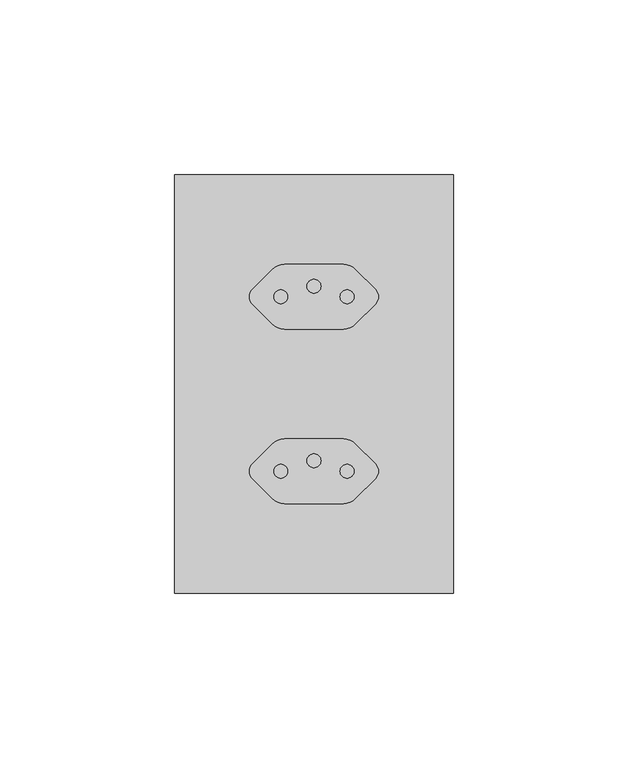
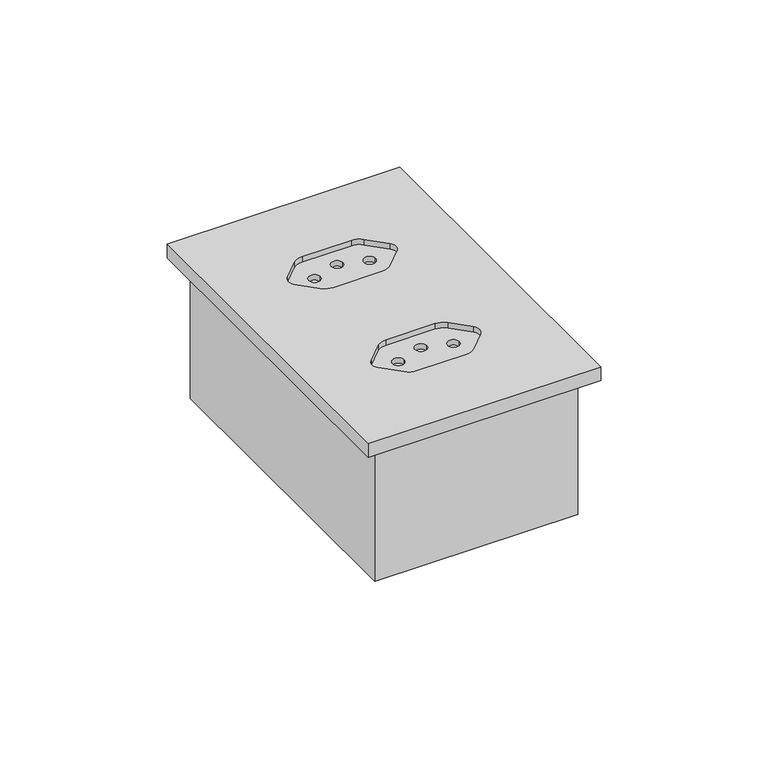
"""IFC4 building model written with IfcOpenShell, lengths in millimetres: proxy geometry, CAIXA VERTICE V7 : Tomada 10A 2s."""

from ifc_helpers import new_model, si_unit, frame, origin, place, context, project, spatial, polyline, circle_curve, faceted_brep, source, transform, mapped, element, save
from ifc_brep_helpers import plane_surface, revolved_surface, advanced_brep


def electrical_fixtures_a300802b(model_context):
    return source(origin(), model_context, "Body", "SolidModel", [
        faceted_brep([(33.0, 247.0, -48.0), (33.0, 353.0, -48.0), (-33.0, 353.0, -48.0), (-33.0, 247.0, -48.0), (35.0, 355.0, -50.0), (35.0, 245.0, -50.0), (-35.0, 245.0, -50.0), (-35.0, 355.0, -50.0), (-35.0, 355.0, 0.0), (35.0, 355.0, 0.0), (-35.0, 245.0, 0.0), (35.0, 245.0, 0.0), (33.0, 353.0, 0.0), (33.0, 247.0, 0.0), (-33.0, 247.0, 0.0), (-33.0, 353.0, 0.0)], [[[0, 1, 2, 3]], [[4, 5, 6, 7]], [[4, 7, 8, 9]], [[8, 7, 6, 10]], [[10, 6, 5, 11]], [[11, 5, 4, 9]], [[9, 8, 10, 11], [12, 13, 14, 15]], [[13, 12, 1, 0]], [[14, 13, 0, 3]], [[15, 14, 3, 2]], [[12, 15, 2, 1]]]),
        advanced_brep(
        [(40.0, 360.0, 5.0), (-40.0, 360.0, 5.0), (-40.0, 240.0, 5.0), (40.0, 240.0, 5.0), (8.4215729, 315.75, 5.0), (-8.4215729, 315.75, 5.0), (-11.9571068, 317.2144661, 5.0), (-17.6213203, 322.8786797, 5.0), (-17.6213203, 327.1213203, 5.0), (-11.9571068, 332.7855339, 5.0), (-8.4215729, 334.25, 5.0), (8.4215729, 334.25, 5.0), (11.9571068, 332.7855339, 5.0), (17.6213203, 327.1213203, 5.0), (17.6213203, 322.8786797, 5.0), (11.9571068, 317.2144661, 5.0), (8.4215729, 265.75, 5.0), (-8.4215729, 265.75, 5.0), (-11.9571068, 267.2144661, 5.0), (-17.6213203, 272.8786797, 5.0), (-17.6213203, 277.1213203, 5.0), (-11.9571068, 282.7855339, 5.0), (-8.4215729, 284.25, 5.0), (8.4215729, 284.25, 5.0), (11.9571068, 282.7855339, 5.0), (17.6213203, 277.1213203, 5.0), (17.6213203, 272.8786797, 5.0), (11.9571068, 267.2144661, 5.0), (-40.0, 360.0, 0.0), (40.0, 360.0, 0.0), (40.0, 240.0, 0.0), (-40.0, 240.0, 0.0), (8.4215729, 315.75, 3.0), (11.9571068, 317.2144661, 3.0), (17.6213203, 322.8786797, 3.0), (17.6213203, 327.1213203, 3.0), (11.9571068, 332.7855339, 3.0), (8.4215729, 334.25, 3.0), (-8.4215729, 334.25, 3.0), (-11.9571068, 332.7855339, 3.0), (-17.6213203, 327.1213203, 3.0), (-17.6213203, 322.8786797, 3.0), (-11.9571068, 317.2144661, 3.0), (-8.4215729, 315.75, 3.0), (-7.5, 325.0, 3.0), (-11.5, 325.0, 3.0), (11.5, 325.0, 3.0), (7.5, 325.0, 3.0), (2.0, 328.0, 3.0), (-2.0, 328.0, 3.0), (-11.5, 325.0, 1.0), (-7.5, 325.0, 1.0), (7.5, 325.0, 1.0), (11.5, 325.0, 1.0), (-2.0, 328.0, 1.0), (2.0, 328.0, 1.0), (8.4215729, 265.75, 3.0), (11.9571068, 267.2144661, 3.0), (17.6213203, 272.8786797, 3.0), (17.6213203, 277.1213203, 3.0), (11.9571068, 282.7855339, 3.0), (8.4215729, 284.25, 3.0), (-8.4215729, 284.25, 3.0), (-11.9571068, 282.7855339, 3.0), (-17.6213203, 277.1213203, 3.0), (-17.6213203, 272.8786797, 3.0), (-11.9571068, 267.2144661, 3.0), (-8.4215729, 265.75, 3.0), (-7.5, 275.0, 3.0), (-11.5, 275.0, 3.0), (11.5, 275.0, 3.0), (7.5, 275.0, 3.0), (2.0, 278.0, 3.0), (-2.0, 278.0, 3.0), (-11.5, 275.0, 1.0), (-7.5, 275.0, 1.0), (7.5, 275.0, 1.0), (11.5, 275.0, 1.0), (-2.0, 278.0, 1.0), (2.0, 278.0, 1.0)],
        [
            (0, 1),
            (1, 2),
            (2, 3),
            (3, 0),
            (4, 5),
            (5, 6, circle_curve(frame((-8.4215729, 320.75, 5.0), z_axis=(0.0, 0.0, -1.0), x_axis=(-1.0, 0.0, 0.0)), 5.0)),
            (6, 7),
            (7, 8, circle_curve(frame((-15.5, 325.0, 5.0), z_axis=(0.0, 0.0, -1.0), x_axis=(-1.0, 0.0, 0.0)), 3.0)),
            (8, 9),
            (9, 10, circle_curve(frame((-8.4215729, 329.25, 5.0), z_axis=(0.0, 0.0, -1.0), x_axis=(-1.0, 0.0, 0.0)), 5.0)),
            (10, 11),
            (11, 12, circle_curve(frame((8.4215729, 329.25, 5.0), z_axis=(0.0, 0.0, -1.0), x_axis=(-1.0, 0.0, 0.0)), 5.0)),
            (12, 13),
            (13, 14, circle_curve(frame((15.5, 325.0, 5.0), z_axis=(0.0, 0.0, -1.0), x_axis=(-1.0, 0.0, 0.0)), 3.0)),
            (14, 15),
            (15, 4, circle_curve(frame((8.4215729, 320.75, 5.0), z_axis=(0.0, 0.0, -1.0), x_axis=(-1.0, 0.0, 0.0)), 5.0)),
            (16, 17),
            (17, 18, circle_curve(frame((-8.4215729, 270.75, 5.0), z_axis=(0.0, 0.0, -1.0), x_axis=(-1.0, 0.0, 0.0)), 5.0)),
            (18, 19),
            (19, 20, circle_curve(frame((-15.5, 275.0, 5.0), z_axis=(0.0, 0.0, -1.0), x_axis=(-1.0, 0.0, 0.0)), 3.0)),
            (20, 21),
            (21, 22, circle_curve(frame((-8.4215729, 279.25, 5.0), z_axis=(0.0, 0.0, -1.0), x_axis=(-1.0, 0.0, 0.0)), 5.0)),
            (22, 23),
            (23, 24, circle_curve(frame((8.4215729, 279.25, 5.0), z_axis=(0.0, 0.0, -1.0), x_axis=(-1.0, 0.0, 0.0)), 5.0)),
            (24, 25),
            (25, 26, circle_curve(frame((15.5, 275.0, 5.0), z_axis=(0.0, 0.0, -1.0), x_axis=(-1.0, 0.0, 0.0)), 3.0)),
            (26, 27),
            (27, 16, circle_curve(frame((8.4215729, 270.75, 5.0), z_axis=(0.0, 0.0, -1.0), x_axis=(-1.0, 0.0, 0.0)), 5.0)),
            (28, 29),
            (29, 30),
            (30, 31),
            (31, 28),
            (0, 29),
            (28, 1),
            (31, 2),
            (30, 3),
            (32, 33, circle_curve(frame((8.4215729, 320.75, 3.0), z_axis=(0.0, 0.0, 1.0), x_axis=(-1.0, 0.0, 0.0)), 5.0)),
            (33, 34),
            (34, 35, circle_curve(frame((15.5, 325.0, 3.0), z_axis=(0.0, 0.0, 1.0), x_axis=(-1.0, 0.0, 0.0)), 3.0)),
            (35, 36),
            (36, 37, circle_curve(frame((8.4215729, 329.25, 3.0), z_axis=(0.0, 0.0, 1.0), x_axis=(-1.0, 0.0, 0.0)), 5.0)),
            (37, 38),
            (38, 39, circle_curve(frame((-8.4215729, 329.25, 3.0), z_axis=(0.0, 0.0, 1.0), x_axis=(-1.0, 0.0, 0.0)), 5.0)),
            (39, 40),
            (40, 41, circle_curve(frame((-15.5, 325.0, 3.0), z_axis=(0.0, 0.0, 1.0), x_axis=(-1.0, 0.0, 0.0)), 3.0)),
            (41, 42),
            (42, 43, circle_curve(frame((-8.4215729, 320.75, 3.0), z_axis=(0.0, 0.0, 1.0), x_axis=(-1.0, 0.0, 0.0)), 5.0)),
            (43, 32),
            (44, 45, circle_curve(frame((-9.5, 325.0, 3.0), z_axis=(0.0, 0.0, -1.0), x_axis=(1.0, 2.301812013077709e-12, 0.0)), 2.0)),
            (45, 44, circle_curve(frame((-9.5, 325.0, 3.0), z_axis=(0.0, 0.0, -1.0), x_axis=(1.0, 2.301812013077709e-12, 0.0)), 2.0)),
            (46, 47, circle_curve(frame((9.5, 325.0, 3.0), z_axis=(0.0, 0.0, -1.0), x_axis=(1.0, 2.301812013077709e-12, 0.0)), 2.0)),
            (47, 46, circle_curve(frame((9.5, 325.0, 3.0), z_axis=(0.0, 0.0, -1.0), x_axis=(1.0, 2.301812013077709e-12, 0.0)), 2.0)),
            (48, 49, circle_curve(frame((0.0, 328.0, 3.0), z_axis=(0.0, 0.0, -1.0), x_axis=(1.0, 2.301812013077709e-12, 0.0)), 2.0)),
            (49, 48, circle_curve(frame((0.0, 328.0, 3.0), z_axis=(0.0, 0.0, -1.0), x_axis=(1.0, 2.301812013077709e-12, 0.0)), 2.0)),
            (43, 5),
            (4, 32),
            (42, 6),
            (41, 7),
            (40, 8),
            (39, 9),
            (38, 10),
            (37, 11),
            (36, 12),
            (35, 13),
            (34, 14),
            (33, 15),
            (50, 51, circle_curve(frame((-9.5, 325.0, 1.0), z_axis=(0.0, 0.0, 1.0), x_axis=(1.0, 2.301812013077709e-12, 0.0)), 2.0)),
            (51, 50, circle_curve(frame((-9.5, 325.0, 1.0), z_axis=(0.0, 0.0, 1.0), x_axis=(1.0, 2.301812013077709e-12, 0.0)), 2.0)),
            (52, 53, circle_curve(frame((9.5, 325.0, 1.0), z_axis=(0.0, 0.0, 1.0), x_axis=(1.0, 2.301812013077709e-12, 0.0)), 2.0)),
            (53, 52, circle_curve(frame((9.5, 325.0, 1.0), z_axis=(0.0, 0.0, 1.0), x_axis=(1.0, 2.301812013077709e-12, 0.0)), 2.0)),
            (54, 55, circle_curve(frame((0.0, 328.0, 1.0), z_axis=(0.0, 0.0, 1.0), x_axis=(1.0, 2.301812013077709e-12, 0.0)), 2.0)),
            (55, 54, circle_curve(frame((0.0, 328.0, 1.0), z_axis=(0.0, 0.0, 1.0), x_axis=(1.0, 2.301812013077709e-12, 0.0)), 2.0)),
            (44, 51),
            (50, 45),
            (46, 53),
            (52, 47),
            (48, 55),
            (54, 49),
            (56, 57, circle_curve(frame((8.4215729, 270.75, 3.0), z_axis=(0.0, 0.0, 1.0), x_axis=(-1.0, 0.0, 0.0)), 5.0)),
            (57, 58),
            (58, 59, circle_curve(frame((15.5, 275.0, 3.0), z_axis=(0.0, 0.0, 1.0), x_axis=(-1.0, 0.0, 0.0)), 3.0)),
            (59, 60),
            (60, 61, circle_curve(frame((8.4215729, 279.25, 3.0), z_axis=(0.0, 0.0, 1.0), x_axis=(-1.0, 0.0, 0.0)), 5.0)),
            (61, 62),
            (62, 63, circle_curve(frame((-8.4215729, 279.25, 3.0), z_axis=(0.0, 0.0, 1.0), x_axis=(-1.0, 0.0, 0.0)), 5.0)),
            (63, 64),
            (64, 65, circle_curve(frame((-15.5, 275.0, 3.0), z_axis=(0.0, 0.0, 1.0), x_axis=(-1.0, 0.0, 0.0)), 3.0)),
            (65, 66),
            (66, 67, circle_curve(frame((-8.4215729, 270.75, 3.0), z_axis=(0.0, 0.0, 1.0), x_axis=(-1.0, 0.0, 0.0)), 5.0)),
            (67, 56),
            (68, 69, circle_curve(frame((-9.5, 275.0, 3.0), z_axis=(0.0, 0.0, -1.0), x_axis=(1.0, 2.301812013077709e-12, 0.0)), 2.0)),
            (69, 68, circle_curve(frame((-9.5, 275.0, 3.0), z_axis=(0.0, 0.0, -1.0), x_axis=(1.0, 2.301812013077709e-12, 0.0)), 2.0)),
            (70, 71, circle_curve(frame((9.5, 275.0, 3.0), z_axis=(0.0, 0.0, -1.0), x_axis=(1.0, 2.301812013077709e-12, 0.0)), 2.0)),
            (71, 70, circle_curve(frame((9.5, 275.0, 3.0), z_axis=(0.0, 0.0, -1.0), x_axis=(1.0, 2.301812013077709e-12, 0.0)), 2.0)),
            (72, 73, circle_curve(frame((0.0, 278.0, 3.0), z_axis=(0.0, 0.0, -1.0), x_axis=(1.0, 2.301812013077709e-12, 0.0)), 2.0)),
            (73, 72, circle_curve(frame((0.0, 278.0, 3.0), z_axis=(0.0, 0.0, -1.0), x_axis=(1.0, 2.301812013077709e-12, 0.0)), 2.0)),
            (67, 17),
            (16, 56),
            (66, 18),
            (65, 19),
            (64, 20),
            (63, 21),
            (62, 22),
            (61, 23),
            (60, 24),
            (59, 25),
            (58, 26),
            (57, 27),
            (74, 75, circle_curve(frame((-9.5, 275.0, 1.0), z_axis=(0.0, 0.0, 1.0), x_axis=(1.0, 2.301812013077709e-12, 0.0)), 2.0)),
            (75, 74, circle_curve(frame((-9.5, 275.0, 1.0), z_axis=(0.0, 0.0, 1.0), x_axis=(1.0, 2.301812013077709e-12, 0.0)), 2.0)),
            (76, 77, circle_curve(frame((9.5, 275.0, 1.0), z_axis=(0.0, 0.0, 1.0), x_axis=(1.0, 2.301812013077709e-12, 0.0)), 2.0)),
            (77, 76, circle_curve(frame((9.5, 275.0, 1.0), z_axis=(0.0, 0.0, 1.0), x_axis=(1.0, 2.301812013077709e-12, 0.0)), 2.0)),
            (78, 79, circle_curve(frame((0.0, 278.0, 1.0), z_axis=(0.0, 0.0, 1.0), x_axis=(1.0, 2.301812013077709e-12, 0.0)), 2.0)),
            (79, 78, circle_curve(frame((0.0, 278.0, 1.0), z_axis=(0.0, 0.0, 1.0), x_axis=(1.0, 2.301812013077709e-12, 0.0)), 2.0)),
            (68, 75),
            (74, 69),
            (70, 77),
            (76, 71),
            (72, 79),
            (78, 73),
        ],
        [
            plane_surface(frame((-60.0, 360.0, 5.0), z_axis=(0.0, 0.0, 1.0), x_axis=(-1.0, 0.0, 0.0))),
            plane_surface(frame((-60.0, 360.0, 0.0), z_axis=(0.0, 0.0, -1.0), x_axis=(1.0, 0.0, 0.0))),
            plane_surface(frame((40.0, 360.0, 5.0), z_axis=(0.0, 1.0, 0.0), x_axis=(0.0, 0.0, -1.0))),
            plane_surface(frame((-40.0, 360.0, 5.0), z_axis=(-1.0, 0.0, 0.0), x_axis=(0.0, 0.0, -1.0))),
            plane_surface(frame((-40.0, 240.0, 5.0), z_axis=(0.0, -1.0, 0.0), x_axis=(0.0, 0.0, -1.0))),
            plane_surface(frame((40.0, 240.0, 5.0), z_axis=(1.0, 0.0, 0.0), x_axis=(0.0, 0.0, -1.0))),
            plane_surface(frame((3.4215729, 320.75, 3.0), z_axis=(0.0, 0.0, 1.0), x_axis=(0.0, 1.0, 0.0))),
            plane_surface(frame((-8.4215729, 315.75, 5.0), z_axis=(0.0, 1.0, 0.0), x_axis=(0.0, 0.0, -1.0))),
            revolved_surface(polyline([(-13.4215729, 320.75, 5.0), (-13.4215729, 320.75, 3.0)]), (-8.4215729, 320.75, 3.0), (0.0, 0.0, 1.0)),
            plane_surface(frame((-17.6213203, 322.8786797, 5.0), z_axis=(0.7071067811865045, 0.7071067811865905, 0.0), x_axis=(0.0, 0.0, -1.0))),
            revolved_surface(polyline([(-18.5, 325.0, 5.0), (-18.5, 325.0, 3.0)]), (-15.5, 325.0, 3.0), (0.0, 0.0, 1.0)),
            plane_surface(frame((-11.9571068, 332.7855339, 5.0), z_axis=(0.7071067811865515, -0.7071067811865437, 0.0), x_axis=(0.0, 0.0, -1.0))),
            revolved_surface(polyline([(-13.4215729, 329.25, 5.0), (-13.4215729, 329.25, 3.0)]), (-8.4215729, 329.25, 3.0), (0.0, 0.0, 1.0)),
            plane_surface(frame((8.4215729, 334.25, 5.0), z_axis=(0.0, -1.0, 0.0), x_axis=(0.0, 0.0, -1.0))),
            revolved_surface(polyline([(3.4215728999999993, 329.25, 5.0), (3.4215728999999993, 329.25, 3.0)]), (8.4215729, 329.25, 3.0), (0.0, 0.0, 1.0)),
            plane_surface(frame((17.6213203, 327.1213203, 5.0), z_axis=(-0.7071067811865307, -0.7071067811865643, 0.0), x_axis=(0.0, 0.0, -1.0))),
            revolved_surface(polyline([(12.5, 325.0, 5.0), (12.5, 325.0, 3.0)]), (15.5, 325.0, 3.0), (0.0, 0.0, 1.0)),
            plane_surface(frame((11.9571068, 317.2144661, 5.0), z_axis=(-0.7071067811865893, 0.7071067811865058, 0.0), x_axis=(0.0, 0.0, -1.0))),
            revolved_surface(polyline([(3.4215728999999993, 320.75, 5.0), (3.4215728999999993, 320.75, 3.0)]), (8.4215729, 320.75, 3.0), (0.0, 0.0, 1.0)),
            plane_surface(frame((-7.5, 325.0, 1.0), z_axis=(0.0, 0.0, 1.0), x_axis=(2.301812013077709e-12, -1.0, 0.0))),
            revolved_surface(polyline([(-7.5, 325.0000000000046, 3.0), (-7.5, 325.0000000000046, 1.0)]), (-9.5, 325.0, 1.0), (0.0, 0.0, 1.0)),
            revolved_surface(polyline([(11.5, 325.0000000000046, 3.0), (11.5, 325.0000000000046, 1.0)]), (9.5, 325.0, 5.0), (0.0, 0.0, 1.0)),
            revolved_surface(polyline([(2.0, 328.0000000000046, 3.0), (2.0, 328.0000000000046, 1.0)]), (0.0, 328.0, 5.0), (0.0, 0.0, 1.0)),
            plane_surface(frame((3.4215729, 270.75, 3.0), z_axis=(0.0, 0.0, 1.0), x_axis=(0.0, 1.0, 0.0))),
            plane_surface(frame((-8.4215729, 265.75, 5.0), z_axis=(0.0, 1.0, 0.0), x_axis=(0.0, 0.0, -1.0))),
            revolved_surface(polyline([(-13.4215729, 270.75, 5.0), (-13.4215729, 270.75, 3.0)]), (-8.4215729, 270.75, 3.0), (0.0, 0.0, 1.0)),
            plane_surface(frame((-17.6213203, 272.8786797, 5.0), z_axis=(0.7071067811865045, 0.7071067811865905, 0.0), x_axis=(0.0, 0.0, -1.0))),
            revolved_surface(polyline([(-18.5, 275.0, 5.0), (-18.5, 275.0, 3.0)]), (-15.5, 275.0, 3.0), (0.0, 0.0, 1.0)),
            plane_surface(frame((-11.9571068, 282.7855339, 5.0), z_axis=(0.7071067811865515, -0.7071067811865437, 0.0), x_axis=(0.0, 0.0, -1.0))),
            revolved_surface(polyline([(-13.4215729, 279.25, 5.0), (-13.4215729, 279.25, 3.0)]), (-8.4215729, 279.25, 3.0), (0.0, 0.0, 1.0)),
            plane_surface(frame((8.4215729, 284.25, 5.0), z_axis=(0.0, -1.0, 0.0), x_axis=(0.0, 0.0, -1.0))),
            revolved_surface(polyline([(3.4215728999999993, 279.25, 5.0), (3.4215728999999993, 279.25, 3.0)]), (8.4215729, 279.25, 3.0), (0.0, 0.0, 1.0)),
            plane_surface(frame((17.6213203, 277.1213203, 5.0), z_axis=(-0.7071067811865307, -0.7071067811865643, 0.0), x_axis=(0.0, 0.0, -1.0))),
            revolved_surface(polyline([(12.5, 275.0, 5.0), (12.5, 275.0, 3.0)]), (15.5, 275.0, 3.0), (0.0, 0.0, 1.0)),
            plane_surface(frame((11.9571068, 267.2144661, 5.0), z_axis=(-0.7071067811865893, 0.7071067811865058, 0.0), x_axis=(0.0, 0.0, -1.0))),
            revolved_surface(polyline([(3.4215728999999993, 270.75, 5.0), (3.4215728999999993, 270.75, 3.0)]), (8.4215729, 270.75, 3.0), (0.0, 0.0, 1.0)),
            plane_surface(frame((-7.5, 275.0, 1.0), z_axis=(0.0, 0.0, 1.0), x_axis=(2.301812013077709e-12, -1.0, 0.0))),
            revolved_surface(polyline([(-7.5, 275.0000000000046, 3.0), (-7.5, 275.0000000000046, 1.0)]), (-9.5, 275.0, 1.0), (0.0, 0.0, 1.0)),
            revolved_surface(polyline([(11.5, 275.0000000000046, 3.0), (11.5, 275.0000000000046, 1.0)]), (9.5, 275.0, 5.0), (0.0, 0.0, 1.0)),
            revolved_surface(polyline([(2.0, 278.0000000000046, 3.0), (2.0, 278.0000000000046, 1.0)]), (0.0, 278.0, 5.0), (0.0, 0.0, 1.0)),
        ],
        [
            (0, [[1, 2, 3, 4], [5, 6, 7, 8, 9, 10, 11, 12, 13, 14, 15, 16], [17, 18, 19, 20, 21, 22, 23, 24, 25, 26, 27, 28]]),
            (1, [[29, 30, 31, 32]]),
            (2, [[-1, 33, -29, 34]]),
            (3, [[-2, -34, -32, 35]]),
            (4, [[-3, -35, -31, 36]]),
            (5, [[-4, -36, -30, -33]]),
            (6, [[37, 38, 39, 40, 41, 42, 43, 44, 45, 46, 47, 48], [49, 50], [51, 52], [53, 54]]),
            (7, [[-48, 55, -5, 56]]),
            (8, [[-47, 57, -6, -55]]),
            (9, [[-46, 58, -7, -57]]),
            (10, [[-45, 59, -8, -58]]),
            (11, [[-44, 60, -9, -59]]),
            (12, [[-43, 61, -10, -60]]),
            (13, [[-42, 62, -11, -61]]),
            (14, [[-41, 63, -12, -62]]),
            (15, [[-40, 64, -13, -63]]),
            (16, [[-39, 65, -14, -64]]),
            (17, [[-38, 66, -15, -65]]),
            (18, [[-37, -56, -16, -66]]),
            (19, [[67, 68]]),
            (19, [[69, 70]]),
            (19, [[71, 72]]),
            (20, [[-49, 73, -67, 74]]),
            (20, [[-50, -74, -68, -73]]),
            (21, [[-51, 75, -69, 76]]),
            (21, [[-52, -76, -70, -75]]),
            (22, [[-53, 77, -71, 78]]),
            (22, [[-54, -78, -72, -77]]),
            (23, [[79, 80, 81, 82, 83, 84, 85, 86, 87, 88, 89, 90], [91, 92], [93, 94], [95, 96]]),
            (24, [[-90, 97, -17, 98]]),
            (25, [[-89, 99, -18, -97]]),
            (26, [[-88, 100, -19, -99]]),
            (27, [[-87, 101, -20, -100]]),
            (28, [[-86, 102, -21, -101]]),
            (29, [[-85, 103, -22, -102]]),
            (30, [[-84, 104, -23, -103]]),
            (31, [[-83, 105, -24, -104]]),
            (32, [[-82, 106, -25, -105]]),
            (33, [[-81, 107, -26, -106]]),
            (34, [[-80, 108, -27, -107]]),
            (35, [[-79, -98, -28, -108]]),
            (36, [[109, 110]]),
            (36, [[111, 112]]),
            (36, [[113, 114]]),
            (37, [[-91, 115, -109, 116]]),
            (37, [[-92, -116, -110, -115]]),
            (38, [[-93, 117, -111, 118]]),
            (38, [[-94, -118, -112, -117]]),
            (39, [[-95, 119, -113, 120]]),
            (39, [[-96, -120, -114, -119]]),
        ],
    ),
    ])


if __name__ == "__main__":
    model = new_model("IFC4")
    model_context = context("Model", 3, world=origin())
    ifc_project = project(units=[si_unit("LENGTHUNIT", "METRE", prefix="MILLI")], contexts=[model_context])
    site = spatial("IfcSite", under=ifc_project)
    building = spatial("IfcBuilding", under=site)
    placement = place(None, origin())
    electrical_fixtures_shape = electrical_fixtures_a300802b(model_context)
    element("IfcBuildingElementProxy", 1, Name="CAIXA VERTICE V7 : Tomada 10A 2s", ObjectType="CAIXA VERTICE V7 : Tomada 10A 2s", at=placement, inside=building, context=model_context, shape_type="MappedRepresentation", body=[
        mapped(electrical_fixtures_shape, transform((0.0, 0.0, 0.0), x_axis=(1.0, 0.0, 0.0), y_axis=(0.0, 1.0, 0.0), z_axis=(0.0, 0.0, 1.0))),
    ])
    save(model, "model.ifc")

# Revit data of these elements
# Type "CAIXA VERTICE V7 : Tomada 10A 2s"
#   URL = "www.facebook.com/verticetreinamentos"
#   SEÇÃO [instance default] = ""
#   Rotação [instance default] = 0.00°
#   LARGURA DA TAMPA = 0.08 m
#   BORDA = 0.01 m
#   ALTURA DE INSTALAÇÃO [instance default] = 1.10 m
#   Distância Anotação [instance default] = 0.0015 m
#   ALTURA DA TAMPA = 0.12 m
#   Vertical [instance default] = yes
#   VER SEÇÃO [instance default] = no
#   SHADE ESQ [instance default] = no
#   SHADE DIR [instance default] = yes
#   HORIZONTAL [instance default] = no
#   ANDAR COM A LEGENDA [instance default] = 0
#   Material Tampa [instance default] = Plástico, branco opaco
#   Caixa = element 1798515
#   Anotação = element 1798529
#   Default Elevation = 0
# Element 1 (IfcBuildingElementProxy, "CAIXA VERTICE V7 : Tomada 10A 2s")
#   ALTURA DE INSTALAÇÃO = 0.30 m
#   SHADE DIR = no
#   Materials on its faces: "Plástico, branco opaco"
# Materials
#   "Plástico, branco opaco": class "Plástico", colour RGB 120 120 120, transparency 0, Description = "Plastic, generic, opaque white", Cost = 0
